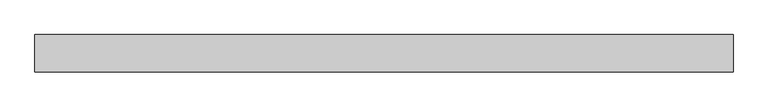
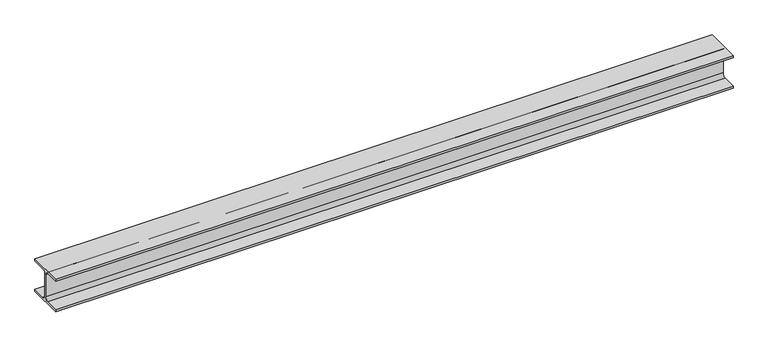
"""IFC4 building model written with IfcOpenShell, lengths in millimetres: beam geometry, NLRS_28_SF_LIB_stalen ligger HEA-AV-CWV-MMBS-SRP_gen_rsf : stalen ligger_gen__HEA 160."""

import ifcopenshell
import ifcopenshell.guid

model = None  # the IFC model being written
_history = None  # IfcOwnerHistory: only IFC2X3 demands one
_inside = {}  # id of a spatial element -> (the spatial element, [elements in it])
_under = {}  # id of a project, library or spatial element -> (it, [spatial elements below it])
_declared = {}  # id of a project -> (the project, [libraries it declares])
_typed = {}  # id of a type object -> (the type object, [elements of that type])
_made_of = {}  # id of a material, layer set ... -> (it, [elements and type objects made of it])


def new_model(schema):
    """Start an empty IFC model of exactly this schema.

    Asked for "IFC4X3", IfcOpenShell would pick the latest addendum, in which some entities
    have other attributes; the version numbers below select the first issue.
    IFC2X3 requires an IfcOwnerHistory on every rooted entity: one is made here for all.
    """
    global model, _history
    if schema == "IFC4X3":
        model = ifcopenshell.file(schema_version=(4, 3, 0, 0))
    else:
        model = ifcopenshell.file(schema=schema)
    _inside.clear()
    _under.clear()
    _declared.clear()
    _typed.clear()
    _made_of.clear()
    _history = None
    if model.schema == "IFC2X3":
        org = make("IfcOrganization", Name="unknown")
        user = make(
            "IfcPersonAndOrganization",
            ThePerson=make("IfcPerson", FamilyName="unknown"),
            TheOrganization=org,
        )
        app = make(
            "IfcApplication",
            ApplicationDeveloper=org,
            Version="unknown",
            ApplicationFullName="unknown",
            ApplicationIdentifier="unknown",
        )
        _history = make(
            "IfcOwnerHistory",
            OwningUser=user,
            OwningApplication=app,
            ChangeAction="ADDED",
            CreationDate=0,
        )
    return model


def make(cls, **values):
    """One entity of the class cls with the attributes given. An attribute that is None is left unset."""
    return model.create_entity(
        cls, **{name: value for name, value in values.items() if value is not None}
    )


def rooted(cls, **values):
    """An entity with a GlobalId (a new one), such as an element, a storey or a relation."""
    return make(cls, GlobalId=ifcopenshell.guid.new(), OwnerHistory=_history, **values)


def si_unit(unit_type, name, prefix=None):
    """IfcSIUnit, for example si_unit("LENGTHUNIT", "METRE", prefix="MILLI")."""
    return make("IfcSIUnit", UnitType=unit_type, Prefix=prefix, Name=name)


def assignment(units):
    """IfcUnitAssignment: the units of a project."""
    return None if units is None else make("IfcUnitAssignment", Units=units)


def point(xyz):
    """IfcCartesianPoint."""
    return None if xyz is None else make("IfcCartesianPoint", Coordinates=xyz)


def direction(xyz):
    """IfcDirection."""
    return None if xyz is None else make("IfcDirection", DirectionRatios=xyz)


def frame(location, z_axis=None, x_axis=None):
    """IfcAxis2Placement3D, a coordinate frame: its origin and axes. An axis left out is left unset."""
    return make(
        "IfcAxis2Placement3D",
        Location=point(location),
        Axis=direction(z_axis),
        RefDirection=direction(x_axis),
    )


def frame_2d(location, x_axis=None):
    """IfcAxis2Placement2D, a coordinate frame in the plane: its origin and x axis."""
    return make(
        "IfcAxis2Placement2D", Location=point(location), RefDirection=direction(x_axis)
    )


def origin():
    """The frame at (0, 0, 0) with its axes left unset."""
    return frame((0.0, 0.0, 0.0))


def place(relative_to, where):
    """IfcLocalPlacement: puts the frame where relative to a parent placement (None: the world)."""
    return make(
        "IfcLocalPlacement", PlacementRelTo=relative_to, RelativePlacement=where
    )


def context(
    kind, dimensions, precision=None, world=None, true_north=None, identifier=None
):
    """IfcGeometricRepresentationContext, for example the 3D "Model" context."""
    return make(
        "IfcGeometricRepresentationContext",
        ContextIdentifier=identifier,
        ContextType=kind,
        CoordinateSpaceDimension=dimensions,
        Precision=precision,
        WorldCoordinateSystem=world,
        TrueNorth=true_north,
    )


def project(units=None, contexts=None):
    """IfcProject with its units and contexts."""
    return rooted(
        "IfcProject",
        Name="project",
        RepresentationContexts=contexts,
        UnitsInContext=assignment(units),
    )


def spatial(cls, under=None, at=None, **own):
    """A site, building, storey or space (cls), placed at a placement, below another one or the project."""
    s = rooted(cls, ObjectPlacement=at, **own)
    if under is not None:
        _under.setdefault(under.id(), (under, []))[1].append(s)
    return s


def polyline(points):
    """IfcPolyline through the points."""
    return make("IfcPolyline", Points=[point(p) for p in points])


def circle_curve(where, radius):
    """IfcCircle in the frame where."""
    return make("IfcCircle", Position=where, Radius=radius)


def trimmed(basis, trim1, trim2, sense, master):
    """IfcTrimmedCurve: the piece of a basis curve between two trims."""
    return make(
        "IfcTrimmedCurve",
        BasisCurve=basis,
        Trim1=trim1,
        Trim2=trim2,
        SenseAgreement=sense,
        MasterRepresentation=master,
    )


def segment(curve, same_sense, transition):
    """IfcCompositeCurveSegment."""
    return make(
        "IfcCompositeCurveSegment",
        Transition=transition,
        SameSense=same_sense,
        ParentCurve=curve,
    )


def composite_curve(segments, self_intersect=None):
    """IfcCompositeCurve: segments joined end to end."""
    return make("IfcCompositeCurve", Segments=segments, SelfIntersect=self_intersect)


def outline(outer, holes=None, kind="AREA"):
    """IfcArbitraryClosedProfileDef: a profile drawn as a closed curve; with holes, ...WithVoids."""
    if holes is None:
        return make("IfcArbitraryClosedProfileDef", ProfileType=kind, OuterCurve=outer)
    return make(
        "IfcArbitraryProfileDefWithVoids",
        ProfileType=kind,
        OuterCurve=outer,
        InnerCurves=holes,
    )


def extrude(swept, where, along, depth):
    """IfcExtrudedAreaSolid: the profile swept, set in the frame where, extruded along a direction by depth."""
    return make(
        "IfcExtrudedAreaSolid",
        SweptArea=swept,
        Position=where,
        ExtrudedDirection=direction(along),
        Depth=depth,
    )


def shape(context_of_items, identifier, shape_type, items):
    """IfcShapeRepresentation: the items that make up one representation, for example the "Body"."""
    return make(
        "IfcShapeRepresentation",
        ContextOfItems=context_of_items,
        RepresentationIdentifier=identifier,
        RepresentationType=shape_type,
        Items=items,
    )


def source(mapping_origin, context_of_items, identifier, shape_type, items):
    """IfcRepresentationMap: a shape defined once, which mapped items show again and again."""
    return make(
        "IfcRepresentationMap",
        MappingOrigin=mapping_origin,
        MappedRepresentation=shape(context_of_items, identifier, shape_type, items),
    )


def transform(
    local_origin,
    x_axis=None,
    y_axis=None,
    z_axis=None,
    scale=None,
    scale2=None,
    scale3=None,
    uniform=True,
):
    """IfcCartesianTransformationOperator3D, or its non-uniform kind. x_axis, y_axis, z_axis: its Axis1, 2, 3."""
    if uniform:
        return make(
            "IfcCartesianTransformationOperator3D",
            Axis1=direction(x_axis),
            Axis2=direction(y_axis),
            LocalOrigin=point(local_origin),
            Scale=scale,
            Axis3=direction(z_axis),
        )
    return make(
        "IfcCartesianTransformationOperator3DnonUniform",
        Axis1=direction(x_axis),
        Axis2=direction(y_axis),
        LocalOrigin=point(local_origin),
        Scale=scale,
        Axis3=direction(z_axis),
        Scale2=scale2,
        Scale3=scale3,
    )


def mapped(mapping_source, mapping_target):
    """IfcMappedItem: shows the shape of a source again, moved by a transform."""
    return make(
        "IfcMappedItem", MappingSource=mapping_source, MappingTarget=mapping_target
    )


def made_of(thing, what):
    """Note that an element or type object is made of a material, layer set ...; save() writes the relation."""
    if what is not None:
        _made_of.setdefault(what.id(), (what, []))[1].append(thing)
    return thing


def element(
    cls,
    number,
    at=None,
    inside=None,
    cuts=None,
    type_object=None,
    material=None,
    context=None,
    identifier="Body",
    shape_type=None,
    held_by="IfcProductDefinitionShape",
    body=None,
    shapes=None,
    **own,
):
    """One element of the class cls, such as IfcWall. Its Tag is "e" and its number.

    at: its placement. inside: the storey or other place that contains it. cuts: it is an
    opening in that element (IfcRelVoidsElement). A single representation is given by context,
    identifier, shape_type and body (its items); several are given by shapes. held_by: the class
    of the entity that holds the representations. save() writes the other relations.
    """
    e = rooted(cls, Tag="e%d" % number, ObjectPlacement=at, **own)
    if body is not None:
        shapes = [shape(context, identifier, shape_type, body)]
    if shapes is not None:
        e.Representation = make(held_by, Representations=shapes)
    if inside is not None:
        _inside.setdefault(inside.id(), (inside, []))[1].append(e)
    if cuts is not None:
        rooted(
            "IfcRelVoidsElement", RelatingBuildingElement=cuts, RelatedOpeningElement=e
        )
    if type_object is not None:
        _typed.setdefault(type_object.id(), (type_object, []))[1].append(e)
    return made_of(e, material)


def aggregate(whole, parts):
    """IfcRelAggregates: a whole, such as a stair, and the parts it consists of."""
    return rooted("IfcRelAggregates", RelatingObject=whole, RelatedObjects=parts)


def save(model, path):
    """Write the relations noted so far, then the file.

    IfcRelAggregates (storeys below a building ...), IfcRelContainedInSpatialStructure (elements
    in a storey), IfcRelDefinesByType, IfcRelAssociatesMaterial and IfcRelDeclares: one each for
    every whole, place, type object, material and project.
    """
    for whole, parts in _under.values():
        aggregate(whole, parts)
    for where, things in _inside.values():
        rooted(
            "IfcRelContainedInSpatialStructure",
            RelatedElements=things,
            RelatingStructure=where,
        )
    for kind, things in _typed.values():
        rooted("IfcRelDefinesByType", RelatedObjects=things, RelatingType=kind)
    for what, things in _made_of.values():
        rooted("IfcRelAssociatesMaterial", RelatedObjects=things, RelatingMaterial=what)
    for by, libraries in _declared.values():
        rooted("IfcRelDeclares", RelatingContext=by, RelatedDefinitions=libraries)
    model.write(path)


def beam_49e60e2e(model_context):
    return source(origin(), model_context, "Body", "SweptSolid", [
        extrude(outline(composite_curve([segment(polyline([(-80.0, 67.0), (-80.0, 76.0), (80.0, 76.0), (80.0, 67.0), (18.0, 67.0)]), True, "CONTINUOUS"), segment(trimmed(circle_curve(frame_2d((18.0, 52.0)), 15.0), [point((18.0, 67.0))], [point((3.0, 52.0))], True, "CARTESIAN"), True, "CONTINUOUS"), segment(polyline([(3.0, 52.0), (3.0, -52.0)]), True, "CONTINUOUS"), segment(trimmed(circle_curve(frame_2d((18.0, -52.0)), 15.0), [point((3.0, -52.0))], [point((18.0, -67.0))], True, "CARTESIAN"), True, "CONTINUOUS"), segment(polyline([(18.0, -67.0), (80.0, -67.0), (80.0, -76.0), (-80.0, -76.0), (-80.0, -67.0), (-18.0, -67.0)]), True, "CONTINUOUS"), segment(trimmed(circle_curve(frame_2d((-18.0, -52.0)), 15.0), [point((-18.0, -67.0))], [point((-3.0, -52.0))], True, "CARTESIAN"), True, "CONTINUOUS"), segment(polyline([(-3.0, -52.0), (-3.0, 52.0)]), True, "CONTINUOUS"), segment(trimmed(circle_curve(frame_2d((-18.0, 52.0)), 15.0), [point((-3.0, 52.0))], [point((-18.0, 67.0))], True, "CARTESIAN"), True, "CONTINUOUS"), segment(polyline([(-18.0, 67.0), (-80.0, 67.0)]), True, "CONTINUOUS")], self_intersect=False)), frame((-1499.9999994, 0.0, 0.0), z_axis=(1.0, 0.0, 0.0), x_axis=(0.0, 1.0, 0.0)), (0.0, 0.0, 1.0), 2999.9999988),
    ])


if __name__ == "__main__":
    model = new_model("IFC4")
    model_context = context("Model", 3, world=origin())
    ifc_project = project(units=[si_unit("LENGTHUNIT", "METRE", prefix="MILLI")], contexts=[model_context])
    site = spatial("IfcSite", under=ifc_project)
    building = spatial("IfcBuilding", under=site)
    placement = place(None, origin())
    beam_shape = beam_49e60e2e(model_context)
    element("IfcBeam", 1, ObjectType="NLRS_28_SF_LIB_stalen ligger HEA-AV-CWV-MMBS-SRP_gen_rsf : stalen ligger_gen__HEA 160", at=placement, inside=building, context=model_context, shape_type="MappedRepresentation", body=[
        mapped(beam_shape, transform((0.0, 0.0, 0.0), x_axis=(1.0, 0.0, 0.0), y_axis=(0.0, 1.0, 0.0), z_axis=(0.0, 0.0, 1.0))),
    ])
    save(model, "model.ifc")

# Revit data of these elements
# Type "NLRS_28_SF_LIB_stalen ligger HEA-AV-CWV-MMBS-SRP_gen_rsf : stalen ligger_gen__HEA 160"
#   Type IfcGUID = "3PFmhy1jzBXho9jMrHR46u"
#   IfcExportAs = "IfcBeamType"
#   Type Comments = "HEA160"
#   Model = " "
#   Manufacturer = " "
#   Fire Rating = " "
#   Description = "stalen ligger HEA160"
#   Assembly Code = "28.11"
#   ra = 15 mm
#   vz = 76 mm
#   vy = 80 mm
#   vpz = 76 mm
#   vpy = 80 mm
#   NLRS_C_lengte [instance default] = 1500 mm
#   Length [instance default] = 1500 mm
#   bf = 160 mm
#   d = 152 mm
#   tf = 9 mm
#   tw = 6 mm
#   Structural Material = NLRS_h2_staal_gen_rsf
#   Keynote = ""
# Element 1 (IfcBeam, "NLRS_28_SF_LIB_stalen ligger HEA-AV-CWV-MMBS-SRP_gen_rsf : stalen ligger_gen__HEA 160")
#   NLRS_C_lengte = 3000 mm
#   Materials on its faces: "NLRS_h2_staal_gen_rsf"
# Materials
#   "NLRS_h2_staal_gen_rsf": class "H - Metaal", colour RGB 189 187 185, transparency 0, Keynote = "h2", Manufacturer = "Revit Standards Foundation", URL = "www.revitstandards.org", Description = "staal", Cost = 0
